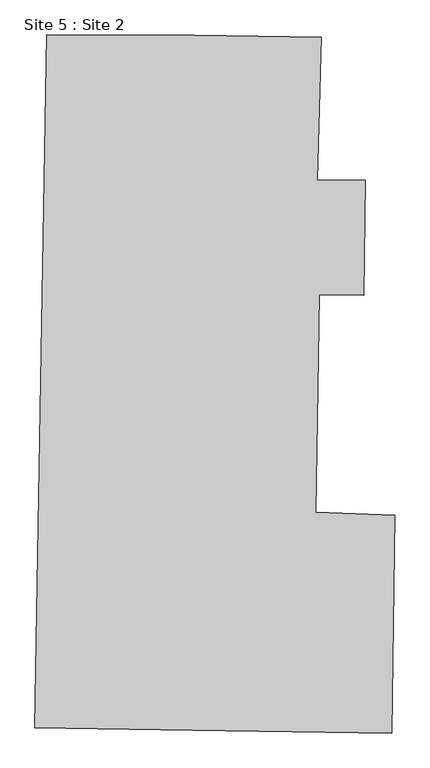
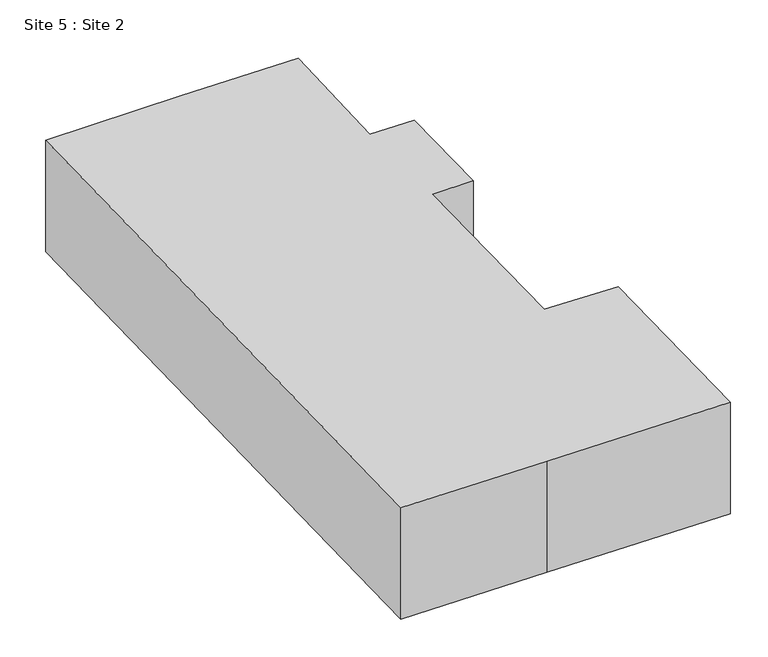
"""IFC4 building model written with IfcOpenShell, lengths in millimetres: geographic element geometry, Site 5 : Site 2."""

from ifc_helpers import new_model, si_unit, frame, origin, place, context, project, spatial, polyline, outline, extrude, source, transform, mapped, element, save


def site_5_site_2_326ef9a9(model_context):
    return source(origin(), model_context, "Body", "SweptSolid", [
        extrude(outline(polyline([(8729.3511309, 115761.4537123), (8505.6065901, 107331.1517319), (11350.1096011, 107289.9427165), (11251.503902, 100483.5629679), (8610.1793752, 100521.8284866), (8423.2700009, 87620.1788693), (13094.9076516, 87450.8912577), (12907.9988905, 74549.2839684), (1123.6383438, 74720.0069008), (-8222.5803931, 74855.4078726), (-7526.4162506, 115895.3465696), (1211.7387515, 115870.3632136), (8729.3511309, 115761.4537123)])), frame((0.0, 0.0, 266395.2), z_axis=(0.0, 0.0, 1.0), x_axis=(1.0, 0.0, 0.0)), (0.0, 0.0, 1.0), 7620.0),
    ])


if __name__ == "__main__":
    model = new_model("IFC4")
    model_context = context("Model", 3, world=origin())
    ifc_project = project(units=[si_unit("LENGTHUNIT", "METRE", prefix="MILLI")], contexts=[model_context])
    site = spatial("IfcSite", under=ifc_project)
    building = spatial("IfcBuilding", under=site)
    placement = place(None, origin())
    site_5_site_2_shape = site_5_site_2_326ef9a9(model_context)
    element("IfcGeographicElement", 1, ObjectType="Site 5 : Site 2", at=placement, inside=building, context=model_context, shape_type="MappedRepresentation", body=[
        mapped(site_5_site_2_shape, transform((0.0, 0.0, 0.0), x_axis=(1.0, 0.0, 0.0), y_axis=(0.0, 1.0, 0.0), z_axis=(0.0, 0.0, 1.0))),
    ])
    save(model, "model.ifc")

# Revit data of these elements
# Element 1 (IfcGeographicElement, "Site 5 : Site 2")
#   Materials on its faces: "EXISTING BUILDING"
# Materials
#   "EXISTING BUILDING": class "Generic", colour RGB 120 120 120, transparency 0, Cost = 0
